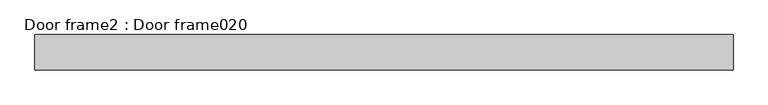
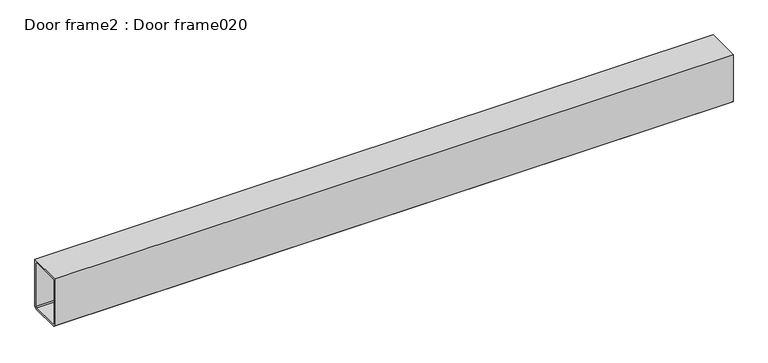
"""IFC4 building model written with IfcOpenShell, lengths in millimetres: proxy geometry, Door frame2 : Door frame020."""

import ifcopenshell
import ifcopenshell.guid

model = None  # the IFC model being written
_history = None  # IfcOwnerHistory: only IFC2X3 demands one
_inside = {}  # id of a spatial element -> (the spatial element, [elements in it])
_under = {}  # id of a project, library or spatial element -> (it, [spatial elements below it])
_declared = {}  # id of a project -> (the project, [libraries it declares])
_typed = {}  # id of a type object -> (the type object, [elements of that type])
_made_of = {}  # id of a material, layer set ... -> (it, [elements and type objects made of it])


def new_model(schema):
    """Start an empty IFC model of exactly this schema.

    Asked for "IFC4X3", IfcOpenShell would pick the latest addendum, in which some entities
    have other attributes; the version numbers below select the first issue.
    IFC2X3 requires an IfcOwnerHistory on every rooted entity: one is made here for all.
    """
    global model, _history
    if schema == "IFC4X3":
        model = ifcopenshell.file(schema_version=(4, 3, 0, 0))
    else:
        model = ifcopenshell.file(schema=schema)
    _inside.clear()
    _under.clear()
    _declared.clear()
    _typed.clear()
    _made_of.clear()
    _history = None
    if model.schema == "IFC2X3":
        org = make("IfcOrganization", Name="unknown")
        user = make(
            "IfcPersonAndOrganization",
            ThePerson=make("IfcPerson", FamilyName="unknown"),
            TheOrganization=org,
        )
        app = make(
            "IfcApplication",
            ApplicationDeveloper=org,
            Version="unknown",
            ApplicationFullName="unknown",
            ApplicationIdentifier="unknown",
        )
        _history = make(
            "IfcOwnerHistory",
            OwningUser=user,
            OwningApplication=app,
            ChangeAction="ADDED",
            CreationDate=0,
        )
    return model


def make(cls, **values):
    """One entity of the class cls with the attributes given. An attribute that is None is left unset."""
    return model.create_entity(
        cls, **{name: value for name, value in values.items() if value is not None}
    )


def rooted(cls, **values):
    """An entity with a GlobalId (a new one), such as an element, a storey or a relation."""
    return make(cls, GlobalId=ifcopenshell.guid.new(), OwnerHistory=_history, **values)


def si_unit(unit_type, name, prefix=None):
    """IfcSIUnit, for example si_unit("LENGTHUNIT", "METRE", prefix="MILLI")."""
    return make("IfcSIUnit", UnitType=unit_type, Prefix=prefix, Name=name)


def assignment(units):
    """IfcUnitAssignment: the units of a project."""
    return None if units is None else make("IfcUnitAssignment", Units=units)


def point(xyz):
    """IfcCartesianPoint."""
    return None if xyz is None else make("IfcCartesianPoint", Coordinates=xyz)


def direction(xyz):
    """IfcDirection."""
    return None if xyz is None else make("IfcDirection", DirectionRatios=xyz)


def frame(location, z_axis=None, x_axis=None):
    """IfcAxis2Placement3D, a coordinate frame: its origin and axes. An axis left out is left unset."""
    return make(
        "IfcAxis2Placement3D",
        Location=point(location),
        Axis=direction(z_axis),
        RefDirection=direction(x_axis),
    )


def origin():
    """The frame at (0, 0, 0) with its axes left unset."""
    return frame((0.0, 0.0, 0.0))


def place(relative_to, where):
    """IfcLocalPlacement: puts the frame where relative to a parent placement (None: the world)."""
    return make(
        "IfcLocalPlacement", PlacementRelTo=relative_to, RelativePlacement=where
    )


def context(
    kind, dimensions, precision=None, world=None, true_north=None, identifier=None
):
    """IfcGeometricRepresentationContext, for example the 3D "Model" context."""
    return make(
        "IfcGeometricRepresentationContext",
        ContextIdentifier=identifier,
        ContextType=kind,
        CoordinateSpaceDimension=dimensions,
        Precision=precision,
        WorldCoordinateSystem=world,
        TrueNorth=true_north,
    )


def project(units=None, contexts=None):
    """IfcProject with its units and contexts."""
    return rooted(
        "IfcProject",
        Name="project",
        RepresentationContexts=contexts,
        UnitsInContext=assignment(units),
    )


def spatial(cls, under=None, at=None, **own):
    """A site, building, storey or space (cls), placed at a placement, below another one or the project."""
    s = rooted(cls, ObjectPlacement=at, **own)
    if under is not None:
        _under.setdefault(under.id(), (under, []))[1].append(s)
    return s


def polyline(points):
    """IfcPolyline through the points."""
    return make("IfcPolyline", Points=[point(p) for p in points])


def outline(outer, holes=None, kind="AREA"):
    """IfcArbitraryClosedProfileDef: a profile drawn as a closed curve; with holes, ...WithVoids."""
    if holes is None:
        return make("IfcArbitraryClosedProfileDef", ProfileType=kind, OuterCurve=outer)
    return make(
        "IfcArbitraryProfileDefWithVoids",
        ProfileType=kind,
        OuterCurve=outer,
        InnerCurves=holes,
    )


def extrude(swept, where, along, depth):
    """IfcExtrudedAreaSolid: the profile swept, set in the frame where, extruded along a direction by depth."""
    return make(
        "IfcExtrudedAreaSolid",
        SweptArea=swept,
        Position=where,
        ExtrudedDirection=direction(along),
        Depth=depth,
    )


def shape(context_of_items, identifier, shape_type, items):
    """IfcShapeRepresentation: the items that make up one representation, for example the "Body"."""
    return make(
        "IfcShapeRepresentation",
        ContextOfItems=context_of_items,
        RepresentationIdentifier=identifier,
        RepresentationType=shape_type,
        Items=items,
    )


def source(mapping_origin, context_of_items, identifier, shape_type, items):
    """IfcRepresentationMap: a shape defined once, which mapped items show again and again."""
    return make(
        "IfcRepresentationMap",
        MappingOrigin=mapping_origin,
        MappedRepresentation=shape(context_of_items, identifier, shape_type, items),
    )


def transform(
    local_origin,
    x_axis=None,
    y_axis=None,
    z_axis=None,
    scale=None,
    scale2=None,
    scale3=None,
    uniform=True,
):
    """IfcCartesianTransformationOperator3D, or its non-uniform kind. x_axis, y_axis, z_axis: its Axis1, 2, 3."""
    if uniform:
        return make(
            "IfcCartesianTransformationOperator3D",
            Axis1=direction(x_axis),
            Axis2=direction(y_axis),
            LocalOrigin=point(local_origin),
            Scale=scale,
            Axis3=direction(z_axis),
        )
    return make(
        "IfcCartesianTransformationOperator3DnonUniform",
        Axis1=direction(x_axis),
        Axis2=direction(y_axis),
        LocalOrigin=point(local_origin),
        Scale=scale,
        Axis3=direction(z_axis),
        Scale2=scale2,
        Scale3=scale3,
    )


def mapped(mapping_source, mapping_target):
    """IfcMappedItem: shows the shape of a source again, moved by a transform."""
    return make(
        "IfcMappedItem", MappingSource=mapping_source, MappingTarget=mapping_target
    )


def made_of(thing, what):
    """Note that an element or type object is made of a material, layer set ...; save() writes the relation."""
    if what is not None:
        _made_of.setdefault(what.id(), (what, []))[1].append(thing)
    return thing


def element(
    cls,
    number,
    at=None,
    inside=None,
    cuts=None,
    type_object=None,
    material=None,
    context=None,
    identifier="Body",
    shape_type=None,
    held_by="IfcProductDefinitionShape",
    body=None,
    shapes=None,
    **own,
):
    """One element of the class cls, such as IfcWall. Its Tag is "e" and its number.

    at: its placement. inside: the storey or other place that contains it. cuts: it is an
    opening in that element (IfcRelVoidsElement). A single representation is given by context,
    identifier, shape_type and body (its items); several are given by shapes. held_by: the class
    of the entity that holds the representations. save() writes the other relations.
    """
    e = rooted(cls, Tag="e%d" % number, ObjectPlacement=at, **own)
    if body is not None:
        shapes = [shape(context, identifier, shape_type, body)]
    if shapes is not None:
        e.Representation = make(held_by, Representations=shapes)
    if inside is not None:
        _inside.setdefault(inside.id(), (inside, []))[1].append(e)
    if cuts is not None:
        rooted(
            "IfcRelVoidsElement", RelatingBuildingElement=cuts, RelatedOpeningElement=e
        )
    if type_object is not None:
        _typed.setdefault(type_object.id(), (type_object, []))[1].append(e)
    return made_of(e, material)


def aggregate(whole, parts):
    """IfcRelAggregates: a whole, such as a stair, and the parts it consists of."""
    return rooted("IfcRelAggregates", RelatingObject=whole, RelatedObjects=parts)


def save(model, path):
    """Write the relations noted so far, then the file.

    IfcRelAggregates (storeys below a building ...), IfcRelContainedInSpatialStructure (elements
    in a storey), IfcRelDefinesByType, IfcRelAssociatesMaterial and IfcRelDeclares: one each for
    every whole, place, type object, material and project.
    """
    for whole, parts in _under.values():
        aggregate(whole, parts)
    for where, things in _inside.values():
        rooted(
            "IfcRelContainedInSpatialStructure",
            RelatedElements=things,
            RelatingStructure=where,
        )
    for kind, things in _typed.values():
        rooted("IfcRelDefinesByType", RelatedObjects=things, RelatingType=kind)
    for what, things in _made_of.values():
        rooted("IfcRelAssociatesMaterial", RelatedObjects=things, RelatingMaterial=what)
    for by, libraries in _declared.values():
        rooted("IfcRelDeclares", RelatingContext=by, RelatedDefinitions=libraries)
    model.write(path)


def door_frame2_door_frame020_938791e3(model_context):
    return source(origin(), model_context, "Body", "SweptSolid", [
        extrude(outline(polyline([(9648.8015375, 37902.896), (9750.4015375, 37902.896), (9750.4015375, 37756.846), (9744.0515375, 37750.496), (9655.1515375, 37750.496), (9648.8015375, 37756.846), (9648.8015375, 37902.896)]), holes=[polyline([(9744.0515375, 37759.4762561), (9744.0515375, 37893.9157439), (9741.4212814, 37896.546), (9657.7817936, 37896.546), (9655.1515375, 37893.9157439), (9655.1515375, 37759.4762561), (9657.7817936, 37756.846), (9741.4212814, 37756.846), (9744.0515375, 37759.4762561)])]), frame((-9232.0719278, 0.0, 0.0), z_axis=(1.0, 0.0, 0.0), x_axis=(0.0, 1.0, 0.0)), (0.0, 0.0, 1.0), 1999.85),
    ])


if __name__ == "__main__":
    model = new_model("IFC4")
    model_context = context("Model", 3, world=origin())
    ifc_project = project(units=[si_unit("LENGTHUNIT", "METRE", prefix="MILLI")], contexts=[model_context])
    site = spatial("IfcSite", under=ifc_project)
    building = spatial("IfcBuilding", under=site)
    placement = place(None, origin())
    door_frame2_door_frame020_shape = door_frame2_door_frame020_938791e3(model_context)
    element("IfcBuildingElementProxy", 1, Name="Door frame2 : Door frame020", ObjectType="Door frame2 : Door frame020", at=placement, inside=building, context=model_context, shape_type="MappedRepresentation", body=[
        mapped(door_frame2_door_frame020_shape, transform((0.0, 0.0, 0.0), x_axis=(1.0, 0.0, 0.0), y_axis=(0.0, 1.0, 0.0), z_axis=(0.0, 0.0, 1.0))),
    ])
    save(model, "model.ifc")

# Revit data of these elements
# Type "Door frame2 : Door frame020"
#   NameOverride = "Door frame020"
# Element 1 (IfcBuildingElementProxy, "Door frame2 : Door frame020")
#   Materials on its faces: "DOOR FRAME: TUBE STEEL PROFILE - METALIZED, PRIMED & PAINTED (COLOR PER ARCHITECT)"
# Materials
#   "DOOR FRAME: TUBE STEEL PROFILE - METALIZED, PRIMED & PAINTED (COLOR PER ARCHITECT)": class "Unassigned", colour RGB 128 128 128, transparency 0, Cost = 0
